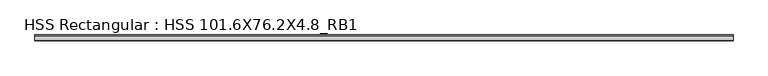
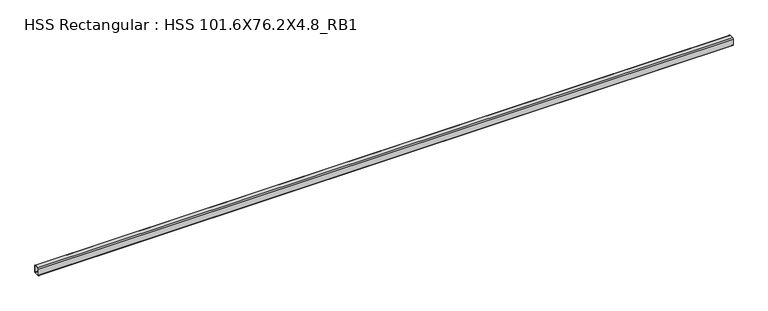
"""IFC4 building model written with IfcOpenShell, lengths in millimetres: beam geometry, HSS Rectangular : HSS 101.6X76.2X4.8_RB1."""

from ifc_helpers import new_model, si_unit, point, frame, frame_2d, origin, place, context, project, spatial, polyline, circle_curve, trimmed, segment, composite_curve, outline, extrude, source, transform, mapped, element, save


def hss_rectangular_hss_101_6x76_2x4_8_rb1_4084155c(model_context):
    return source(origin(), model_context, "Body", "SweptSolid", [
        extrude(outline(composite_curve([segment(polyline([(38.1, 41.275), (38.1, -41.275)]), True, "CONTINUOUS"), segment(trimmed(circle_curve(frame_2d((28.575, -41.275)), 9.525), [point((38.1, -41.275))], [point((28.575, -50.8))], False, "CARTESIAN"), True, "CONTINUOUS"), segment(polyline([(28.575, -50.8), (-28.575, -50.8)]), True, "CONTINUOUS"), segment(trimmed(circle_curve(frame_2d((-28.575, -41.275)), 9.525), [point((-28.575, -50.8))], [point((-38.1, -41.275))], False, "CARTESIAN"), True, "CONTINUOUS"), segment(polyline([(-38.1, -41.275), (-38.1, 41.275)]), True, "CONTINUOUS"), segment(trimmed(circle_curve(frame_2d((-28.575, 41.275)), 9.525), [point((-38.1, 41.275))], [point((-28.575, 50.8))], False, "CARTESIAN"), True, "CONTINUOUS"), segment(polyline([(-28.575, 50.8), (28.575, 50.8)]), True, "CONTINUOUS"), segment(trimmed(circle_curve(frame_2d((28.575, 41.275)), 9.525), [point((28.575, 50.8))], [point((38.1, 41.275))], False, "CARTESIAN"), True, "CONTINUOUS")], self_intersect=False), holes=[composite_curve([segment(trimmed(circle_curve(frame_2d((-28.575, 41.275)), 4.7625), [point((-28.575, 46.0375))], [point((-33.3375, 41.275))], True, "CARTESIAN"), True, "CONTINUOUS"), segment(polyline([(-33.3375, 41.275), (-33.3375, -41.275)]), True, "CONTINUOUS"), segment(trimmed(circle_curve(frame_2d((-28.575, -41.275)), 4.7625), [point((-33.3375, -41.275))], [point((-28.575, -46.0375))], True, "CARTESIAN"), True, "CONTINUOUS"), segment(polyline([(-28.575, -46.0375), (28.575, -46.0375)]), True, "CONTINUOUS"), segment(trimmed(circle_curve(frame_2d((28.575, -41.275)), 4.7625), [point((28.575, -46.0375))], [point((33.3375, -41.275))], True, "CARTESIAN"), True, "CONTINUOUS"), segment(polyline([(33.3375, -41.275), (33.3375, 41.275)]), True, "CONTINUOUS"), segment(trimmed(circle_curve(frame_2d((28.575, 41.275)), 4.7625), [point((33.3375, 41.275))], [point((28.575, 46.0375))], True, "CARTESIAN"), True, "CONTINUOUS"), segment(polyline([(28.575, 46.0375), (-28.575, 46.0375)]), True, "CONTINUOUS")], self_intersect=False)]), frame((-10485.4915, 0.0, 0.0), z_axis=(1.0, 0.0, 0.0), x_axis=(0.0, 1.0, 0.0)), (0.0, 0.0, 1.0), 8946.546177),
    ])


if __name__ == "__main__":
    model = new_model("IFC4")
    model_context = context("Model", 3, world=origin())
    ifc_project = project(units=[si_unit("LENGTHUNIT", "METRE", prefix="MILLI")], contexts=[model_context])
    site = spatial("IfcSite", under=ifc_project)
    building = spatial("IfcBuilding", under=site)
    placement = place(None, origin())
    hss_rectangular_hss_101_6x76_2x4_8_rb1_shape = hss_rectangular_hss_101_6x76_2x4_8_rb1_4084155c(model_context)
    element("IfcBeam", 1, ObjectType="HSS Rectangular : HSS 101.6X76.2X4.8_RB1", at=placement, inside=building, context=model_context, shape_type="MappedRepresentation", body=[
        mapped(hss_rectangular_hss_101_6x76_2x4_8_rb1_shape, transform((0.0, 0.0, 0.0), x_axis=(1.0, 0.0, 0.0), y_axis=(0.0, 1.0, 0.0), z_axis=(0.0, 0.0, 1.0))),
    ])
    save(model, "model.ifc")

# Revit data of these elements
# Type "HSS Rectangular : HSS 101.6X76.2X4.8_RB1"
#   Section Name Key = "HSS 4X3X3/16"
#   Assembly Code = "B10"
#   Width = 7.62 cm
#   Wall Nominal Thickness = 0.4763 cm
#   Wall Design Thickness = 0.442 cm
#   Torsional Moment of Inertia = 260.561 cm⁴
#   Torsional Modulus = 61.2876 cm³
#   Section Area = 14.4516 cm²
#   Plastic Modulus weak axis = 40.3122 cm³
#   Plastic Modulus strong axis = 49.1612 cm³
#   Perimeter = 0.881482 m²/m
#   Outer Fillet = 0.9525 cm
#   Nominal Weight = 12.1285 kgf/m
#   Moment of Inertia weak axis = 131.529 cm⁴
#   Moment of Inertia strong axis = 205.202 cm⁴
#   Inner Fillet = 0.4763 cm
#   Height = 10.16 cm
#   Elastic Modulus weak axis = 34.4128 cm³
#   Elastic Modulus strong axis = 40.476 cm³
#   Centroid Vertical = 5.08 cm
#   Centroid Horizontal = 3.81 cm
#   Length [instance default] = 1524 mm
#   Structural Material [instance default] = Steel ASTM A500, Grade B, Rectangular and Square
#   Principal Axes Angle = 0
# Element 1 (IfcBeam, "HSS Rectangular : HSS 101.6X76.2X4.8_RB1")
#   Structural Material = Steel ASTM A992
#   Materials on its faces: "Steel ASTM A992"
# Materials
#   "Steel ASTM A500, Grade B, Rectangular and Square": class "Metal", colour RGB 199 199 199, transparency 0, Description = "Carbon steel", Cost = 0
#   "Steel ASTM A992": class "Metal", colour RGB 199 199 199, transparency 0, Description = "Structural steel 50ksi", Cost = 0
